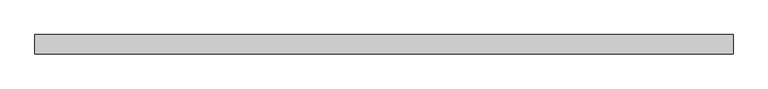
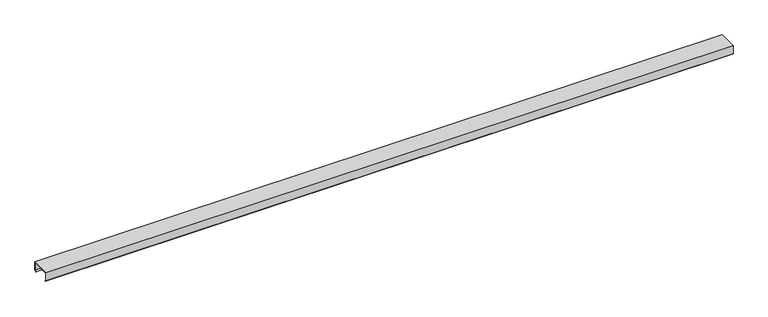
"""IFC4 building model written with IfcOpenShell, lengths in millimetres: proxy geometry, Generic Models 7:Generic Models 1:1:Generic Models 1:1 : Generic Models 7:Generic Models 1:337419:17 : Generic Models 7:Generic Models 1:1:Generic Models 1:1 : Generic Models 7:Generic Models 1:337419:306201."""

from ifc_helpers import new_model, si_unit, frame, origin, place, context, project, spatial, polyline, outline, extrude, source, transform, mapped, element, save


def generic_models_0e7b4f9b(model_context):
    return source(origin(), model_context, "Body", "SweptSolid", [
        extrude(outline(polyline([(-578797.4913841, 6128.940625), (-578797.4913841, 6040.040625), (-578812.0845307, 6027.7955211), (-578813.870275, 6029.9236883), (-578800.2695091, 6041.336086), (-578800.2695091, 6126.1625), (-578997.9132591, 6126.1625), (-578997.9132591, 6041.336086), (-578984.3124931, 6029.9236883), (-578986.0982374, 6027.7955211), (-579000.6913841, 6040.040625), (-579000.6913841, 6128.940625), (-578797.4913841, 6128.940625)])), frame((574430.911724, 0.0, 0.0), z_axis=(1.0, 0.0, 0.0), x_axis=(0.0, 1.0, 0.0)), (0.0, 0.0, 1.0), 7315.2),
    ])


if __name__ == "__main__":
    model = new_model("IFC4")
    model_context = context("Model", 3, world=origin())
    ifc_project = project(units=[si_unit("LENGTHUNIT", "METRE", prefix="MILLI")], contexts=[model_context])
    site = spatial("IfcSite", under=ifc_project)
    building = spatial("IfcBuilding", under=site)
    placement = place(None, origin())
    generic_models_shape = generic_models_0e7b4f9b(model_context)
    element("IfcBuildingElementProxy", 1, Name="Generic Models 7:Generic Models 1:1:Generic Models 1:1 : Generic Models 7:Generic Models 1:337419:17 : Generic Models 7:Generic Models 1:1:Generic Models 1:1 : Generic Models 7:Generic Models 1:337419:306201", ObjectType="Generic Models 7:Generic Models 1:1:Generic Models 1:1 : Generic Models 7:Generic Models 1:337419:17 : Generic Models 7:Generic Models 1:1:Generic Models 1:1 : Generic Models 7:Generic Models 1:337419:306201", at=placement, inside=building, context=model_context, shape_type="MappedRepresentation", body=[
        mapped(generic_models_shape, transform((0.0, 0.0, 0.0), x_axis=(1.0, 0.0, 0.0), y_axis=(0.0, 1.0, 0.0), z_axis=(0.0, 0.0, 1.0))),
    ])
    save(model, "model.ifc")

# Revit data of these elements
# Type "Generic Models 7:Generic Models 1:1:Generic Models 1:1 : Generic Models 7:Generic Models 1:337419:17 : Generic Models 7:Generic Models 1:1:Generic Models 1:1 : Generic Models 7:Generic Models 1:337419:306201"
#   NameOverride = "Generic Models 7:Generic Models 1:1:Generic Models 1:1 : Generic Models 7:Generic Models 1:337419:306201"
#   ObjectTypeOverride = "Generic Models 1:1 : Generic Models 7:Generic Models 1:337419"
#   Reference = "Generic Models 1"
#   Tag = "306201"
# Element 1 (IfcBuildingElementProxy, "Generic Models 7:Generic Models 1:1:Generic Models 1:1 : Generic Models 7:Generic Models 1:337419:17 : Generic Models 7:Generic Models 1:1:Generic Models 1:1 : Generic Models 7:Generic Models 1:337419:306201")
#   Materials on its faces: "'ZEE' SECTION (8.0x3.5Z - SEE STRUCT. DWGS)"
# Materials
#   "'ZEE' SECTION (8.0x3.5Z - SEE STRUCT. DWGS)": class "Unassigned", colour RGB 210 209 208, transparency 0, Keynote = "M05121300.02", Cost = 0
